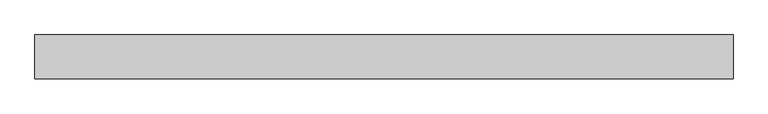
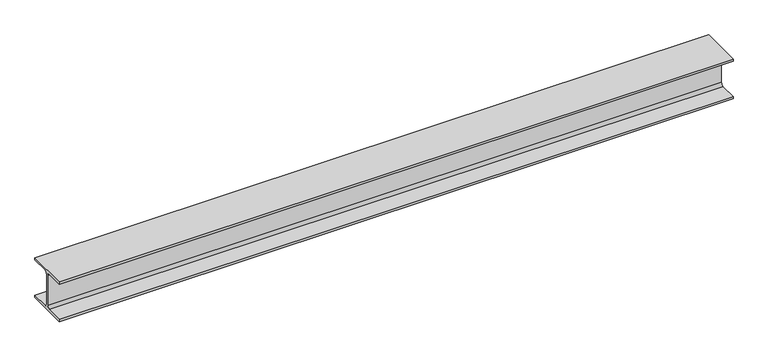
"""IFC4 building model written with IfcOpenShell, lengths in millimetres: beam geometry, 0912_Steel Framing_H-KSD3502 : H_SB_ASB_H-200x200x8x12."""

from ifc_helpers import new_model, si_unit, point, frame, frame_2d, origin, place, context, project, spatial, polyline, circle_curve, trimmed, segment, composite_curve, outline, extrude, source, transform, mapped, element, save


def beam_a3f8eec5(model_context):
    return source(origin(), model_context, "Body", "SweptSolid", [
        extrude(outline(composite_curve([segment(polyline([(100.0, -88.0), (100.0, -100.0), (-100.0, -100.0), (-100.0, -88.0), (-17.0, -88.0)]), True, "CONTINUOUS"), segment(trimmed(circle_curve(frame_2d((-17.0, -75.0)), 13.0), [point((-17.0, -88.0))], [point((-4.0, -75.0))], True, "CARTESIAN"), True, "CONTINUOUS"), segment(polyline([(-4.0, -75.0), (-4.0, 75.0)]), True, "CONTINUOUS"), segment(trimmed(circle_curve(frame_2d((-17.0, 75.0)), 13.0), [point((-4.0, 75.0))], [point((-17.0, 88.0))], True, "CARTESIAN"), True, "CONTINUOUS"), segment(polyline([(-17.0, 88.0), (-100.0, 88.0), (-100.0, 100.0), (100.0, 100.0), (100.0, 88.0), (17.0, 88.0)]), True, "CONTINUOUS"), segment(trimmed(circle_curve(frame_2d((17.0, 75.0)), 13.0), [point((17.0, 88.0))], [point((4.0, 75.0))], True, "CARTESIAN"), True, "CONTINUOUS"), segment(polyline([(4.0, 75.0), (4.0, -75.0)]), True, "CONTINUOUS"), segment(trimmed(circle_curve(frame_2d((17.0, -75.0)), 13.0), [point((4.0, -75.0))], [point((17.0, -88.0))], True, "CARTESIAN"), True, "CONTINUOUS"), segment(polyline([(17.0, -88.0), (100.0, -88.0)]), True, "CONTINUOUS")], self_intersect=False)), frame((-1386.1214584, 0.0, 0.0), z_axis=(1.0, 0.0, 0.0), x_axis=(0.0, 1.0, 0.0)), (0.0, 0.0, 1.0), 3195.9813864),
    ])


if __name__ == "__main__":
    model = new_model("IFC4")
    model_context = context("Model", 3, world=origin())
    ifc_project = project(units=[si_unit("LENGTHUNIT", "METRE", prefix="MILLI")], contexts=[model_context])
    site = spatial("IfcSite", under=ifc_project)
    building = spatial("IfcBuilding", under=site)
    placement = place(None, origin())
    beam_shape = beam_a3f8eec5(model_context)
    element("IfcBeam", 1, ObjectType="0912_Steel Framing_H-KSD3502 : H_SB_ASB_H-200x200x8x12", at=placement, inside=building, context=model_context, shape_type="MappedRepresentation", body=[
        mapped(beam_shape, transform((0.0, 0.0, 0.0), x_axis=(1.0, 0.0, 0.0), y_axis=(0.0, 1.0, 0.0), z_axis=(0.0, 0.0, 1.0))),
    ])
    save(model, "model.ifc")

# Revit data of these elements
# Type "0912_Steel Framing_H-KSD3502 : H_SB_ASB_H-200x200x8x12"
#   H_WM Code_1 = "S01AA002-00001 | Main Steel Structure Fabrication Work | Shelter/Building | Medium Steel - Standard (90KG/M>Weight≥30KG/M) | Material: (   )"
#   H_WM Code_2 = "S03AA028-00001 | Main Steel Structure Erection Work | Shelter/Building | Medium Steel (90KG/M>Weight≥30KG/M) | Material: (   )"
#   H_WM Code_3 = "S01AA010-00001 | Main Steel Structure Fabrication Work | Shelter/Building | Steel Painting/Coating | for Non-Fireproofed Steel Surface, Surface Preparation, Primer, Second & Final Coat | Material: (   )"
#   H_Q'ty Cal Type Tag = "SB-Q2"
#   Width = 20.0 cm
#   Web Thickness = 0.8 cm
#   Web Fillet = 1.3 cm
#   Warping Constant = 141000.0 cm⁶
#   W = 0
#   Torsional Moment of Inertia = 26.2485 cm⁴
#   Section Area = 63.53 cm²
#   Plastic Modulus weak axis = 244.0 cm³
#   Plastic Modulus strong axis = 525.0 cm³
#   Perimeter = 1.16 m²/m
#   Nominal Weight = 49.90 kgf/m
#   Moment of Inertia weak axis = 1600.00 cm⁴
#   Moment of Inertia strong axis = 4720.00 cm⁴
#   Height = 20.0 cm
#   Flange Thickness = 1.2 cm
#   Elastic Modulus weak axis = 160.0 cm³
#   Elastic Modulus strong axis = 472.0 cm³
#   Centroid Vertical = 10.0 cm
#   Centroid Horizontal = 10.0 cm
#   Ix = 47200000
#   Length [instance default] = 1.5240 m
#   Zx = 525000
#   b = 0.2000 m
#   h = 0.2000 m
#   r = 0.0130 m
#   s = 0.0080 m
#   t = 0.0120 m
#   A = 0.006353 m²
#   Structural Material [instance default] = Steel, 45-345
#   Assembly Code = ""
# Element 1 (IfcBeam, "0912_Steel Framing_H-KSD3502 : H_SB_ASB_H-200x200x8x12")
#   Structural Material = none
# Materials
#   "Steel, 45-345": class "Metal", colour RGB 189 187 185, transparency 0, Description = "Steel 345 MPa", Cost = 0
